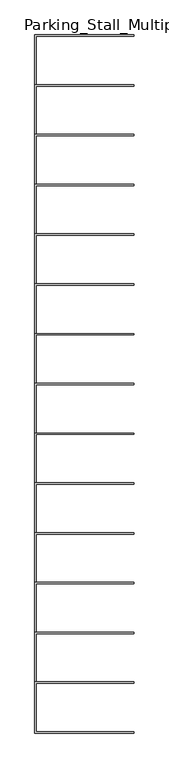
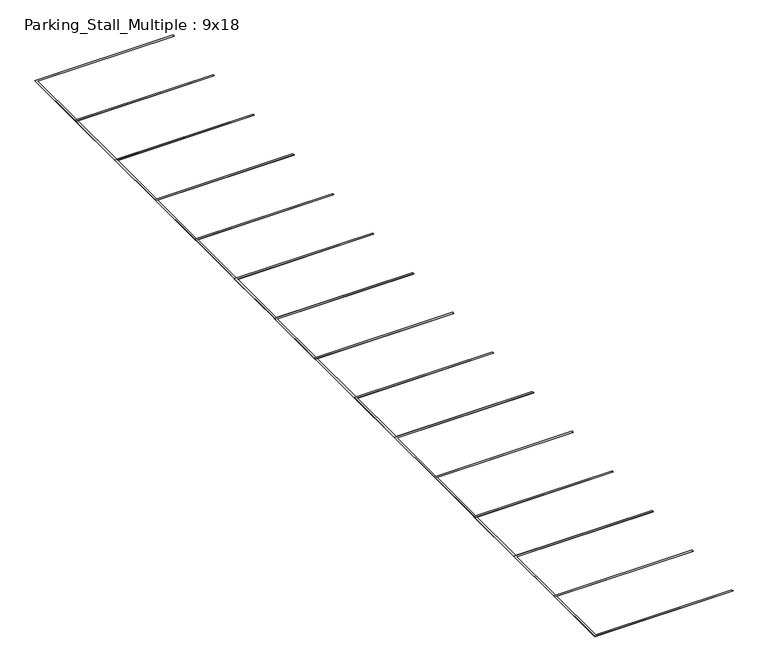
"""IFC4 building model written with IfcOpenShell, lengths in millimetres: proxy geometry, Parking_Stall_Multiple : 9x18."""

from ifc_helpers import new_model, si_unit, origin, origin_with_axes, place, context, project, spatial, polyline, outline, extrude, source, transform, mapped, element, save


def parking_stall_multiple_9x18_fcf1a113(model_context):
    return source(origin(), model_context, "Body", "SweptSolid", [
        extrude(outline(polyline([(5486.4, -35661.6), (5486.4, -35737.8), (76.2, -35737.8), (76.2, -38404.8), (5486.4, -38404.8), (5486.4, -38481.0), (0.0, -38481.0), (0.0, -35661.6), (5486.4, -35661.6)])), origin_with_axes(), (0.0, 0.0, 1.0), 6.35),
        extrude(outline(polyline([(5486.4, -32918.4), (5486.4, -32994.6), (76.2, -32994.6), (76.2, -35661.6), (5486.4, -35661.6), (5486.4, -35737.8), (0.0, -35737.8), (0.0, -32918.4), (5486.4, -32918.4)])), origin_with_axes(), (0.0, 0.0, 1.0), 6.35),
        extrude(outline(polyline([(5486.4, -30175.2), (5486.4, -30251.4), (76.2, -30251.4), (76.2, -32918.4), (5486.4, -32918.4), (5486.4, -32994.6), (0.0, -32994.6), (0.0, -30175.2), (5486.4, -30175.2)])), origin_with_axes(), (0.0, 0.0, 1.0), 6.35),
        extrude(outline(polyline([(5486.4, -27432.0), (5486.4, -27508.2), (76.2, -27508.2), (76.2, -30175.2), (5486.4, -30175.2), (5486.4, -30251.4), (0.0, -30251.4), (0.0, -27432.0), (5486.4, -27432.0)])), origin_with_axes(), (0.0, 0.0, 1.0), 6.35),
        extrude(outline(polyline([(5486.4, -24688.8), (5486.4, -24765.0), (76.2, -24765.0), (76.2, -27432.0), (5486.4, -27432.0), (5486.4, -27508.2), (0.0, -27508.2), (0.0, -24688.8), (5486.4, -24688.8)])), origin_with_axes(), (0.0, 0.0, 1.0), 6.35),
        extrude(outline(polyline([(5486.4, -21945.6), (5486.4, -22021.8), (76.2, -22021.8), (76.2, -24688.8), (5486.4, -24688.8), (5486.4, -24765.0), (0.0, -24765.0), (0.0, -21945.6), (5486.4, -21945.6)])), origin_with_axes(), (0.0, 0.0, 1.0), 6.35),
        extrude(outline(polyline([(5486.4, -19202.4), (5486.4, -19278.6), (76.2, -19278.6), (76.2, -21945.6), (5486.4, -21945.6), (5486.4, -22021.8), (0.0, -22021.8), (0.0, -19202.4), (5486.4, -19202.4)])), origin_with_axes(), (0.0, 0.0, 1.0), 6.35),
        extrude(outline(polyline([(5486.4, -16459.2), (5486.4, -16535.4), (76.2, -16535.4), (76.2, -19202.4), (5486.4, -19202.4), (5486.4, -19278.6), (0.0, -19278.6), (0.0, -16459.2), (5486.4, -16459.2)])), origin_with_axes(), (0.0, 0.0, 1.0), 6.35),
        extrude(outline(polyline([(5486.4, -13716.0), (5486.4, -13792.2), (76.2, -13792.2), (76.2, -16459.2), (5486.4, -16459.2), (5486.4, -16535.4), (0.0, -16535.4), (0.0, -13716.0), (5486.4, -13716.0)])), origin_with_axes(), (0.0, 0.0, 1.0), 6.35),
        extrude(outline(polyline([(5486.4, -10972.8), (5486.4, -11049.0), (76.2, -11049.0), (76.2, -13716.0), (5486.4, -13716.0), (5486.4, -13792.2), (0.0, -13792.2), (0.0, -10972.8), (5486.4, -10972.8)])), origin_with_axes(), (0.0, 0.0, 1.0), 6.35),
        extrude(outline(polyline([(5486.4, -8229.6), (5486.4, -8305.8), (76.2, -8305.8), (76.2, -10972.8), (5486.4, -10972.8), (5486.4, -11049.0), (0.0, -11049.0), (0.0, -8229.6), (5486.4, -8229.6)])), origin_with_axes(), (0.0, 0.0, 1.0), 6.35),
        extrude(outline(polyline([(5486.4, -5486.4), (5486.4, -5562.6), (76.2, -5562.6), (76.2, -8229.6), (5486.4, -8229.6), (5486.4, -8305.8), (0.0, -8305.8), (0.0, -5486.4), (5486.4, -5486.4)])), origin_with_axes(), (0.0, 0.0, 1.0), 6.35),
        extrude(outline(polyline([(5486.4, -2743.2), (5486.4, -2819.4), (76.2, -2819.4), (76.2, -5486.4), (5486.4, -5486.4), (5486.4, -5562.6), (0.0, -5562.6), (0.0, -2743.2), (5486.4, -2743.2)])), origin_with_axes(), (0.0, 0.0, 1.0), 6.35),
        extrude(outline(polyline([(5486.4, 0.0), (5486.4, -76.2), (76.2, -76.2), (76.2, -2743.2), (5486.4, -2743.2), (5486.4, -2819.4), (0.0, -2819.4), (0.0, 0.0), (5486.4, 0.0)])), origin_with_axes(), (0.0, 0.0, 1.0), 6.35),
    ])


if __name__ == "__main__":
    model = new_model("IFC4")
    model_context = context("Model", 3, world=origin())
    ifc_project = project(units=[si_unit("LENGTHUNIT", "METRE", prefix="MILLI")], contexts=[model_context])
    site = spatial("IfcSite", under=ifc_project)
    building = spatial("IfcBuilding", under=site)
    placement = place(None, origin())
    parking_stall_multiple_9x18_shape = parking_stall_multiple_9x18_fcf1a113(model_context)
    element("IfcBuildingElementProxy", 1, Name="Parking_Stall_Multiple : 9x18", ObjectType="Parking_Stall_Multiple : 9x18", at=placement, inside=building, context=model_context, shape_type="MappedRepresentation", body=[
        mapped(parking_stall_multiple_9x18_shape, transform((0.0, 0.0, 0.0), x_axis=(1.0, 0.0, 0.0), y_axis=(0.0, 1.0, 0.0), z_axis=(0.0, 0.0, 1.0))),
    ])
    save(model, "model.ifc")

# Revit data of these elements
# Type "Parking_Stall_Multiple : 9x18"
#   Parking_Width_M = 9' - 0"
#   Parking_Run_Length [instance default] = 65' - 0"
#   Parking_Line_Width = 0' - 3"
#   Parking_Length_M = 18' - 0"
#   Single_Parking_Visibility [instance default] = no
#   Parking_ADA_Symbol = no
#   ParkingUnitsArray [instance default] = 7
#   ParkingUnits [instance default] = 7
#   Multiple_Parking_Visibility [instance default] = yes
#   Parking_Line_Material = none
# Element 1 (IfcBuildingElementProxy, "Parking_Stall_Multiple : 9x18")
#   Parking_Run_Length = 126' - 7.17448"
#   ParkingUnitsArray = 14
#   ParkingUnits = 14
